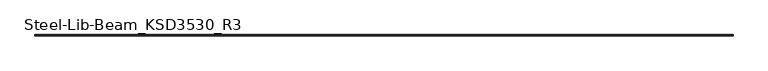
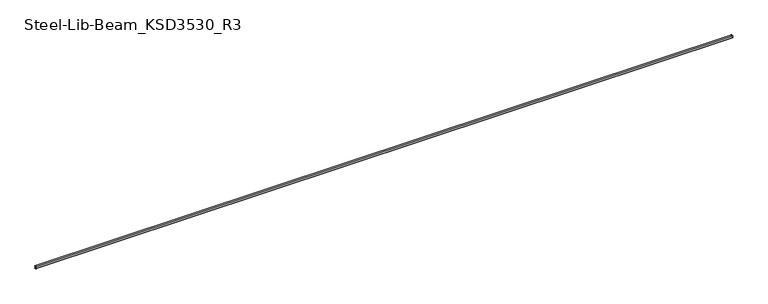
"""IFC4 building model written with IfcOpenShell, lengths in millimetres: beam geometry, Steel-Lib-Beam_KSD3530_R3 : BMS291_C-150×75x20x4.5."""

from ifc_helpers import new_model, si_unit, point, frame, frame_2d, origin, place, context, project, spatial, polyline, circle_curve, trimmed, segment, composite_curve, outline, extrude, source, transform, mapped, element, save


def steel_lib_beam_ksd3530_r3_ac782bcf(model_context):
    return source(origin(), model_context, "Body", "SweptSolid", [
        extrude(outline(composite_curve([segment(polyline([(50.0, 66.0), (50.0, 55.0), (45.5, 55.0), (45.5, 66.0)]), True, "CONTINUOUS"), segment(trimmed(circle_curve(frame_2d((41.0, 66.0)), 4.5), [point((45.5, 66.0))], [point((41.0, 70.5))], True, "CARTESIAN"), True, "CONTINUOUS"), segment(polyline([(41.0, 70.5), (-16.0, 70.5)]), True, "CONTINUOUS"), segment(trimmed(circle_curve(frame_2d((-16.0, 66.0)), 4.5), [point((-16.0, 70.5))], [point((-20.5, 66.0))], True, "CARTESIAN"), True, "CONTINUOUS"), segment(polyline([(-20.5, 66.0), (-20.5, -66.0)]), True, "CONTINUOUS"), segment(trimmed(circle_curve(frame_2d((-16.0, -66.0)), 4.5), [point((-20.5, -66.0))], [point((-16.0, -70.5))], True, "CARTESIAN"), True, "CONTINUOUS"), segment(polyline([(-16.0, -70.5), (41.0, -70.5)]), True, "CONTINUOUS"), segment(trimmed(circle_curve(frame_2d((41.0, -66.0)), 4.5), [point((41.0, -70.5))], [point((45.5, -66.0))], True, "CARTESIAN"), True, "CONTINUOUS"), segment(polyline([(45.5, -66.0), (45.5, -55.0), (50.0, -55.0), (50.0, -66.0)]), True, "CONTINUOUS"), segment(trimmed(circle_curve(frame_2d((41.0, -66.0)), 9.0), [point((50.0, -66.0))], [point((41.0, -75.0))], False, "CARTESIAN"), True, "CONTINUOUS"), segment(polyline([(41.0, -75.0), (-16.0, -75.0)]), True, "CONTINUOUS"), segment(trimmed(circle_curve(frame_2d((-16.0, -66.0)), 9.0), [point((-16.0, -75.0))], [point((-25.0, -66.0))], False, "CARTESIAN"), True, "CONTINUOUS"), segment(polyline([(-25.0, -66.0), (-25.0, 66.0)]), True, "CONTINUOUS"), segment(trimmed(circle_curve(frame_2d((-16.0, 66.0)), 9.0), [point((-25.0, 66.0))], [point((-16.0, 75.0))], False, "CARTESIAN"), True, "CONTINUOUS"), segment(polyline([(-16.0, 75.0), (41.0, 75.0)]), True, "CONTINUOUS"), segment(trimmed(circle_curve(frame_2d((41.0, 66.0)), 9.0), [point((41.0, 75.0))], [point((50.0, 66.0))], False, "CARTESIAN"), True, "CONTINUOUS")], self_intersect=False)), frame((-20450.0, 0.0, 0.0), z_axis=(1.0, 0.0, 0.0), x_axis=(0.0, 1.0, 0.0)), (0.0, 0.0, 1.0), 40900.0),
    ])


if __name__ == "__main__":
    model = new_model("IFC4")
    model_context = context("Model", 3, world=origin())
    ifc_project = project(units=[si_unit("LENGTHUNIT", "METRE", prefix="MILLI")], contexts=[model_context])
    site = spatial("IfcSite", under=ifc_project)
    building = spatial("IfcBuilding", under=site)
    placement = place(None, origin())
    steel_lib_beam_ksd3530_r3_shape = steel_lib_beam_ksd3530_r3_ac782bcf(model_context)
    element("IfcBeam", 1, ObjectType="Steel-Lib-Beam_KSD3530_R3 : BMS291_C-150×75x20x4.5", at=placement, inside=building, context=model_context, shape_type="MappedRepresentation", body=[
        mapped(steel_lib_beam_ksd3530_r3_shape, transform((0.0, 0.0, 0.0), x_axis=(1.0, 0.0, 0.0), y_axis=(0.0, 1.0, 0.0), z_axis=(0.0, 0.0, 1.0))),
    ])
    save(model, "model.ifc")

# Revit data of these elements
# Type "Steel-Lib-Beam_KSD3530_R3 : BMS291_C-150×75x20x4.5"
#   Keynote = "C-150×75x20x4.5"
#   SteelWeight = "Light"
#   x = 0.0250 m
#   t1 = 0.0090 m
#   t = 0.0045 m
#   Surface Area = 0.629834 m²/m
#   Section Area = 13.9688 cm²
#   Mass per Unit Length = 10.9655 kg/m
#   C = 0.0200 m
#   A = 0.0750 m
#   Length [instance default] = 1.5000 m
#   H = 0.1500 m
#   hec_material4 [instance default] = none
#   hec_material3 [instance default] = none
#   hec_material2 [instance default] = none
#   hec_material1 [instance default] = none
#   Structural Material [instance default] = Metal - Steel - Light Gauge
#   Assembly Code = ""
# Element 1 (IfcBeam, "Steel-Lib-Beam_KSD3530_R3 : BMS291_C-150×75x20x4.5")
#   Structural Material = none
# Materials
#   "Metal - Steel - Light Gauge": class "Metal", colour RGB 247 247 247, transparency 0
